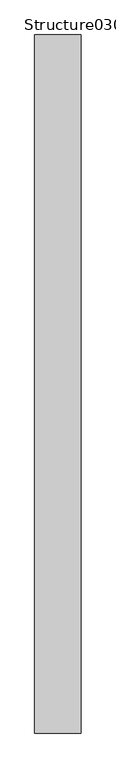
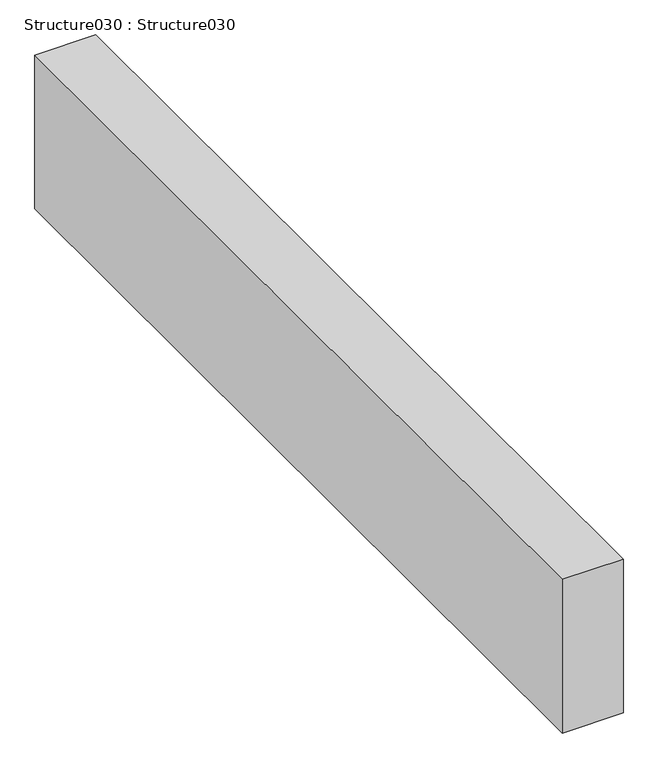
"""IFC4 building model written with IfcOpenShell, lengths in millimetres: proxy geometry, Structure030 : Structure030."""

from ifc_helpers import new_model, si_unit, frame, origin, place, context, project, spatial, polyline, outline, extrude, source, transform, mapped, element, save


def structure030_structure030_d0e04d85(model_context):
    return source(origin(), model_context, "Body", "SweptSolid", [
        extrude(outline(polyline([(-7089.7776325, 7982.1531721), (-7223.1276325, 7982.1531721), (-7223.1276325, 9982.1531721), (-7089.7776325, 9982.1531721), (-7089.7776325, 7982.1531721)])), frame((0.0, 0.0, 39579.2960083), z_axis=(0.0, 0.0, 1.0), x_axis=(1.0, 0.0, 0.0)), (0.0, 0.0, 1.0), 355.6),
    ])


if __name__ == "__main__":
    model = new_model("IFC4")
    model_context = context("Model", 3, world=origin())
    ifc_project = project(units=[si_unit("LENGTHUNIT", "METRE", prefix="MILLI")], contexts=[model_context])
    site = spatial("IfcSite", under=ifc_project)
    building = spatial("IfcBuilding", under=site)
    placement = place(None, origin())
    structure030_structure030_shape = structure030_structure030_d0e04d85(model_context)
    element("IfcBuildingElementProxy", 1, Name="Structure030 : Structure030", ObjectType="Structure030 : Structure030", at=placement, inside=building, context=model_context, shape_type="MappedRepresentation", body=[
        mapped(structure030_structure030_shape, transform((0.0, 0.0, 0.0), x_axis=(1.0, 0.0, 0.0), y_axis=(0.0, 1.0, 0.0), z_axis=(0.0, 0.0, 1.0))),
    ])
    save(model, "model.ifc")

# Revit data of these elements
# Type "Structure030 : Structure030"
#   NameOverride = "Structure030"
# Element 1 (IfcBuildingElementProxy, "Structure030 : Structure030")
#   Materials on its faces: "STRUCTURAL MEMBER (SEE STRUCTURAL DWGS)"
# Materials
#   "STRUCTURAL MEMBER (SEE STRUCTURAL DWGS)": class "Unassigned", colour RGB 176 134 95, transparency 0, Cost = 0
